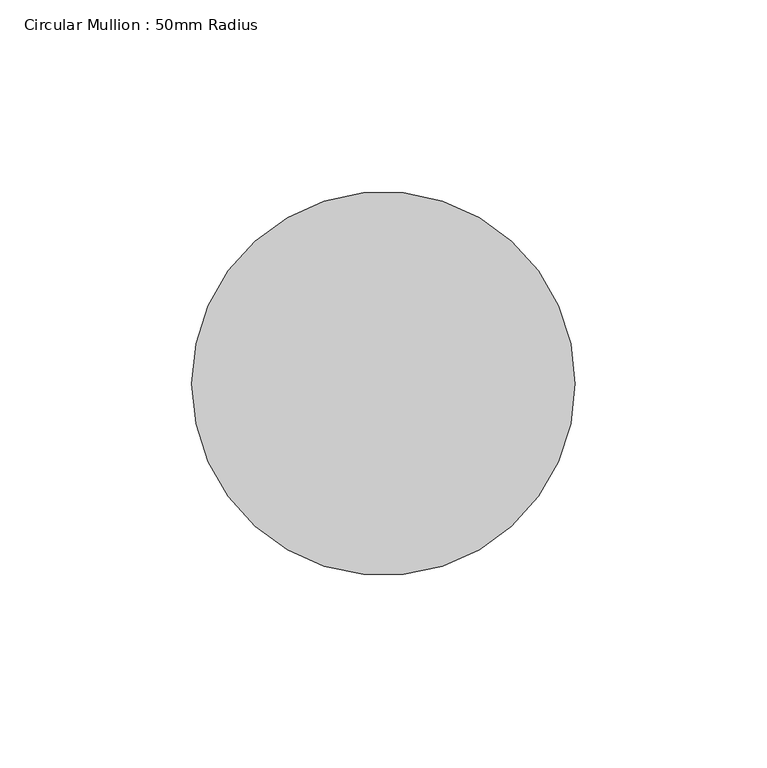
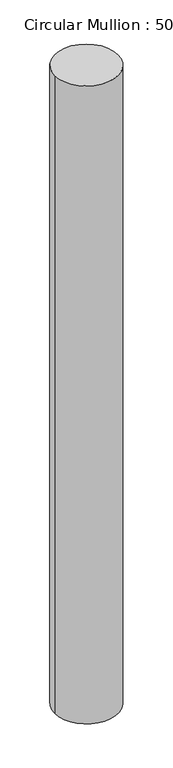
"""IFC4 building model written with IfcOpenShell, lengths in millimetres: member geometry, Circular Mullion : 50mm Radius."""

from ifc_helpers import new_model, si_unit, point, frame, origin, origin_2d, place, context, project, spatial, circle_curve, trimmed, segment, composite_curve, outline, extrude, source, transform, mapped, element, save


def circular_mullion_50mm_radius_dbd5fa57(model_context):
    return source(origin(), model_context, "Body", "SweptSolid", [
        extrude(outline(composite_curve([segment(trimmed(circle_curve(origin_2d(), 50.0), [point((50.0, 0.0))], [point((-50.0, 0.0))], False, "CARTESIAN"), True, "CONTINUOUS"), segment(trimmed(circle_curve(origin_2d(), 50.0), [point((-50.0, 0.0))], [point((50.0, 0.0))], False, "CARTESIAN"), True, "CONTINUOUS")], self_intersect=False)), frame((0.0, 0.0, -1067.1544563), z_axis=(0.0, 0.0, 1.0), x_axis=(1.0, 0.0, 0.0)), (0.0, 0.0, 1.0), 1067.1544563),
    ])


if __name__ == "__main__":
    model = new_model("IFC4")
    model_context = context("Model", 3, world=origin())
    ifc_project = project(units=[si_unit("LENGTHUNIT", "METRE", prefix="MILLI")], contexts=[model_context])
    site = spatial("IfcSite", under=ifc_project)
    building = spatial("IfcBuilding", under=site)
    placement = place(None, origin())
    circular_mullion_50mm_radius_shape = circular_mullion_50mm_radius_dbd5fa57(model_context)
    element("IfcMember", 1, ObjectType="Circular Mullion : 50mm Radius", at=placement, inside=building, context=model_context, shape_type="MappedRepresentation", body=[
        mapped(circular_mullion_50mm_radius_shape, transform((0.0, 0.0, 0.0), x_axis=(1.0, 0.0, 0.0), y_axis=(0.0, 1.0, 0.0), z_axis=(0.0, 0.0, 1.0))),
    ])
    save(model, "model.ifc")

# Revit data of these elements
# Type "Circular Mullion : 50mm Radius"
#   built-in parameter 1007350 = 0.164042 (stored number, unit not read)
# Element 1 (IfcMember, "Circular Mullion : 50mm Radius")
#   Materials on its faces: "Aluminium"
# Materials
#   "Aluminium": class "Metal", colour RGB 247 247 247, transparency 0, Description = "Aluminium 6061", Cost = 0
